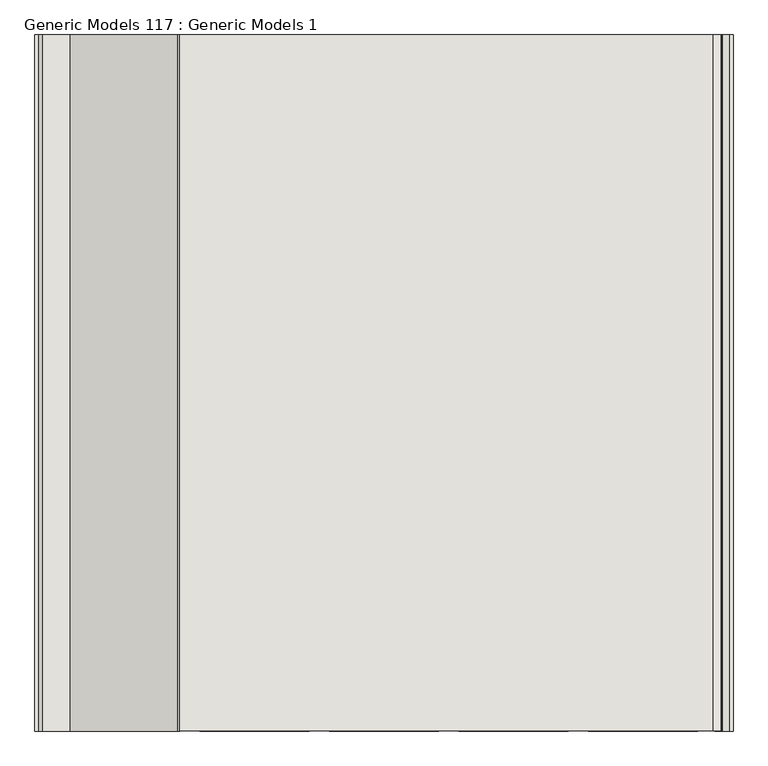
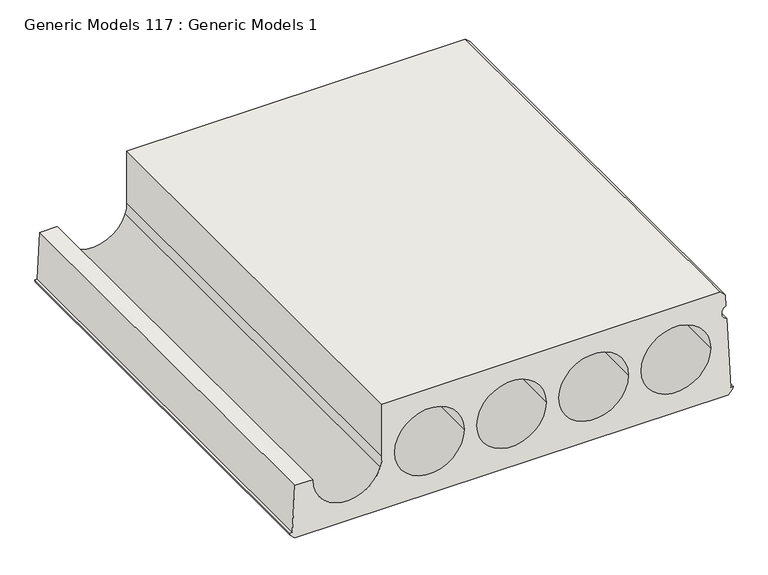
"""IFC4 building model written with IfcOpenShell, lengths in millimetres: wall geometry, Generic Models 117 : Generic Models 1."""

from ifc_helpers import new_model, si_unit, point, frame, frame_2d, origin, place, context, project, spatial, polyline, circle_curve, trimmed, segment, composite_curve, outline, extrude, source, transform, mapped, element, save


def generic_models_117_generic_models_1_ccd83e45(model_context):
    return source(origin(), model_context, "Body", "SweptSolid", [
        extrude(outline(composite_curve([segment(polyline([(2248.1999739, 374822.3375014), (2254.1999619, 374823.0375), (2254.1999619, 374817.037512), (2457.6133066, 374805.2133227)]), True, "CONTINUOUS"), segment(trimmed(circle_curve(frame_2d((2477.0193199, 374811.6399604)), 20.4424809), [point((2457.6133066, 374805.2133227))], [point((2495.5499999, 374803.0081053))], True, "CARTESIAN"), True, "CONTINUOUS"), segment(polyline([(2495.5499999, 374803.0081053), (2527.3000253, 374801.162512), (2539.9999999, 374788.4625374), (2539.9999999, 373859.425), (2387.5999999, 373859.425)]), True, "CONTINUOUS"), segment(trimmed(circle_curve(frame_2d((2387.5999999, 373764.175)), 95.25), [point((2387.5999999, 373859.425))], [point((2360.0836351, 373855.3638818))], True, "CARTESIAN"), True, "CONTINUOUS"), segment(trimmed(circle_curve(frame_2d((2387.5999999, 373764.175)), 95.25), [point((2360.0836351, 373855.3638818))], [point((2387.5999999, 373668.925))], True, "CARTESIAN"), True, "CONTINUOUS"), segment(polyline([(2387.5999999, 373668.925), (2387.5999999, 373620.7668824), (2254.1999619, 373613.012488), (2254.1999619, 373607.0125), (2248.1999739, 373607.7124986), (2235.1999999, 373620.7124726), (2235.1999999, 374809.3375274), (2248.1999739, 374822.3375014)]), True, "CONTINUOUS")], self_intersect=False), holes=[composite_curve([segment(trimmed(circle_curve(frame_2d((2387.5999999, 374665.875)), 95.25), [point((2387.5999999, 374570.625))], [point((2387.5999999, 374761.125))], True, "CARTESIAN"), True, "CONTINUOUS"), segment(trimmed(circle_curve(frame_2d((2387.5999999, 374665.875)), 95.25), [point((2387.5999999, 374761.125))], [point((2387.5999999, 374570.625))], True, "CARTESIAN"), True, "CONTINUOUS")], self_intersect=False), composite_curve([segment(trimmed(circle_curve(frame_2d((2387.5999999, 374215.025)), 95.25), [point((2387.5999999, 374310.275))], [point((2387.5999999, 374119.775))], True, "CARTESIAN"), True, "CONTINUOUS"), segment(trimmed(circle_curve(frame_2d((2387.5999999, 374215.025)), 95.25), [point((2387.5999999, 374119.775))], [point((2387.5999999, 374310.275))], True, "CARTESIAN"), True, "CONTINUOUS")], self_intersect=False), composite_curve([segment(trimmed(circle_curve(frame_2d((2387.5999999, 374440.45)), 95.25), [point((2387.5999999, 374535.7))], [point((2387.5999999, 374345.2))], True, "CARTESIAN"), True, "CONTINUOUS"), segment(trimmed(circle_curve(frame_2d((2387.5999999, 374440.45)), 95.25), [point((2387.5999999, 374345.2))], [point((2387.5999999, 374535.7))], True, "CARTESIAN"), True, "CONTINUOUS")], self_intersect=False), composite_curve([segment(trimmed(circle_curve(frame_2d((2387.5999999, 373989.6)), 95.25), [point((2387.5999999, 373894.35))], [point((2387.5999999, 374084.85))], True, "CARTESIAN"), True, "CONTINUOUS"), segment(trimmed(circle_curve(frame_2d((2387.5999999, 373989.6)), 95.25), [point((2387.5999999, 374084.85))], [point((2387.5999999, 373894.35))], True, "CARTESIAN"), True, "CONTINUOUS")], self_intersect=False)]), frame((0.0, -686.1747735, 0.0), z_axis=(0.0, 1.0, 0.0), x_axis=(0.0, 0.0, 1.0)), (0.0, 0.0, 1.0), 1212.3817147),
    ])


if __name__ == "__main__":
    model = new_model("IFC4")
    model_context = context("Model", 3, world=origin())
    ifc_project = project(units=[si_unit("LENGTHUNIT", "METRE", prefix="MILLI")], contexts=[model_context])
    site = spatial("IfcSite", under=ifc_project)
    building = spatial("IfcBuilding", under=site)
    placement = place(None, origin())
    generic_models_117_generic_models_1_shape = generic_models_117_generic_models_1_ccd83e45(model_context)
    element("IfcWall", 1, ObjectType="Generic Models 117 : Generic Models 1", at=placement, inside=building, context=model_context, shape_type="MappedRepresentation", body=[
        mapped(generic_models_117_generic_models_1_shape, transform((0.0, 0.0, 0.0), x_axis=(1.0, 0.0, 0.0), y_axis=(0.0, 1.0, 0.0), z_axis=(0.0, 0.0, 1.0))),
    ])
    save(model, "model.ifc")

# Revit data of these elements
# Element 1 (IfcWall, "Generic Models 117 : Generic Models 1")
#   Materials on its faces: "PRECAST PLANK - SEE PRECAST SHOPS FOR SIZE"
# Materials
#   "PRECAST PLANK - SEE PRECAST SHOPS FOR SIZE": class "Concrete", colour RGB 191 191 191, transparency 0, Description = "Cast-in-place concrete", Cost = 0
